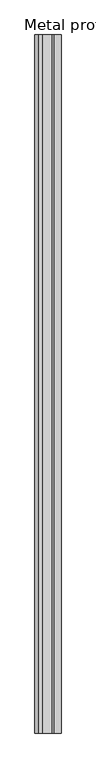
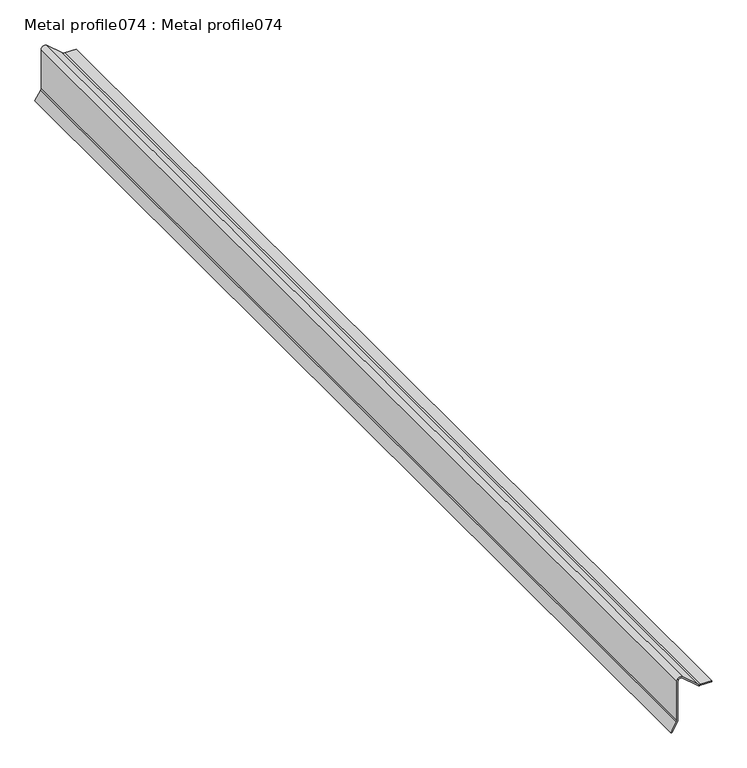
"""IFC4 building model written with IfcOpenShell, lengths in millimetres: proxy geometry, Metal profile074 : Metal profile074."""

from ifc_helpers import new_model, si_unit, point, frame, frame_2d, origin, place, context, project, spatial, polyline, circle_curve, trimmed, segment, composite_curve, outline, extrude, source, transform, mapped, element, save


def metal_profile074_metal_profile074_9453f65b(model_context):
    return source(origin(), model_context, "Body", "SweptSolid", [
        extrude(outline(composite_curve([segment(trimmed(circle_curve(frame_2d((40173.6742187, -9878.6140229)), 6.35), [point((40167.3242187, -9878.6140229))], [point((40168.8617194, -9882.7567696))], True, "CARTESIAN"), True, "CONTINUOUS"), segment(polyline([(40168.8617194, -9882.7567696), (40193.006585, -9910.8051048)]), True, "CONTINUOUS"), segment(trimmed(circle_curve(frame_2d((40188.1940856, -9914.9478516)), 6.35), [point((40193.006585, -9910.8051048))], [point((40188.1940856, -9921.2978516))], False, "CARTESIAN"), True, "CONTINUOUS"), segment(polyline([(40188.1940856, -9921.2978516), (40113.9784377, -9921.2978516)]), True, "CONTINUOUS"), segment(trimmed(circle_curve(frame_2d((40113.9784377, -9927.6478516)), 6.35), [point((40113.9784377, -9921.2978516))], [point((40110.6358579, -9922.248809))], True, "CARTESIAN"), True, "CONTINUOUS"), segment(polyline([(40110.6358579, -9922.248809), (40093.8632812, -9932.6328125), (40092.8105002, -9930.9323267), (40109.5830768, -9920.5483232)]), True, "CONTINUOUS"), segment(trimmed(circle_curve(frame_2d((40113.9784377, -9927.6478516)), 8.35), [point((40109.5830768, -9920.5483232))], [point((40113.9784377, -9919.2978516))], False, "CARTESIAN"), True, "CONTINUOUS"), segment(polyline([(40113.9784377, -9919.2978516), (40188.1940856, -9919.2978516)]), True, "CONTINUOUS"), segment(trimmed(circle_curve(frame_2d((40188.1940856, -9914.9478516)), 4.35), [point((40188.1940856, -9919.2978516))], [point((40191.4908371, -9912.109907))], True, "CARTESIAN"), True, "CONTINUOUS"), segment(polyline([(40191.4908371, -9912.109907), (40167.3459716, -9884.0615717)]), True, "CONTINUOUS"), segment(trimmed(circle_curve(frame_2d((40173.6742187, -9878.6140229)), 8.35), [point((40167.3459716, -9884.0615717))], [point((40165.3242187, -9878.6140229))], False, "CARTESIAN"), True, "CONTINUOUS"), segment(polyline([(40165.3242187, -9878.6140229), (40165.3242188, -9857.6464844), (40167.3242187, -9857.6464844), (40167.3242187, -9878.6140229)]), True, "CONTINUOUS")], self_intersect=False)), frame((0.0, 7982.1531721, 0.0), z_axis=(0.0, 1.0, 0.0), x_axis=(0.0, 0.0, 1.0)), (0.0, 0.0, 1.0), 2000.0),
    ])


if __name__ == "__main__":
    model = new_model("IFC4")
    model_context = context("Model", 3, world=origin())
    ifc_project = project(units=[si_unit("LENGTHUNIT", "METRE", prefix="MILLI")], contexts=[model_context])
    site = spatial("IfcSite", under=ifc_project)
    building = spatial("IfcBuilding", under=site)
    placement = place(None, origin())
    metal_profile074_metal_profile074_shape = metal_profile074_metal_profile074_9453f65b(model_context)
    element("IfcBuildingElementProxy", 1, Name="Metal profile074 : Metal profile074", ObjectType="Metal profile074 : Metal profile074", at=placement, inside=building, context=model_context, shape_type="MappedRepresentation", body=[
        mapped(metal_profile074_metal_profile074_shape, transform((0.0, 0.0, 0.0), x_axis=(1.0, 0.0, 0.0), y_axis=(0.0, 1.0, 0.0), z_axis=(0.0, 0.0, 1.0))),
    ])
    save(model, "model.ifc")

# Revit data of these elements
# Type "Metal profile074 : Metal profile074"
#   NameOverride = "Metal profile074"
# Element 1 (IfcBuildingElementProxy, "Metal profile074 : Metal profile074")
#   Materials on its faces: "ANGLE TRIM"
# Materials
#   "ANGLE TRIM": class "Unassigned", colour RGB 250 255 0, transparency 0
